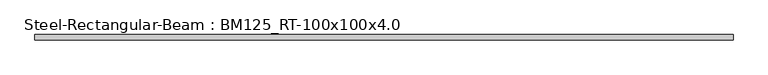
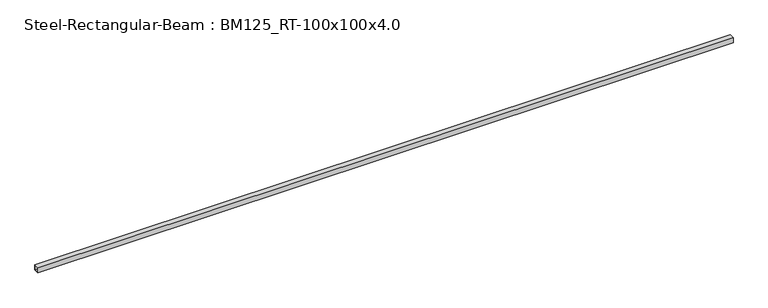
"""IFC4 building model written with IfcOpenShell, lengths in millimetres: beam geometry, Steel-Rectangular-Beam : BM125_RT-100x100x4.0."""

from ifc_helpers import new_model, si_unit, frame, origin, place, context, project, spatial, polyline, outline, extrude, source, transform, mapped, element, save


def steel_rectangular_beam_bm125_rt_100x100x4_0_2c93a6f0(model_context):
    return source(origin(), model_context, "Body", "SweptSolid", [
        extrude(outline(polyline([(-50.0, 50.0), (50.0, 50.0), (50.0, -50.0), (-50.0, -50.0), (-50.0, 50.0)]), holes=[polyline([(46.0, -46.0), (46.0, 46.0), (-46.0, 46.0), (-46.0, -46.0), (46.0, -46.0)])]), frame((-6550.0, 0.0, 0.0), z_axis=(1.0, 0.0, 0.0), x_axis=(0.0, 1.0, 0.0)), (0.0, 0.0, 1.0), 13100.0),
        extrude(outline(polyline([(-50.0, 50.0), (50.0, 50.0), (50.0, -50.0), (-50.0, -50.0), (-50.0, 50.0)]), holes=[polyline([(46.0, -46.0), (46.0, 46.0), (-46.0, 46.0), (-46.0, -46.0), (46.0, -46.0)])]), frame((-6550.0, 0.0, 0.0), z_axis=(1.0, 0.0, 0.0), x_axis=(0.0, 1.0, 0.0)), (0.0, 0.0, 1.0), 13100.0),
        extrude(outline(polyline([(-50.0, 50.0), (50.0, 50.0), (50.0, -50.0), (-50.0, -50.0), (-50.0, 50.0)]), holes=[polyline([(46.0, -46.0), (46.0, 46.0), (-46.0, 46.0), (-46.0, -46.0), (46.0, -46.0)])]), frame((-6550.0, 0.0, 0.0), z_axis=(1.0, 0.0, 0.0), x_axis=(0.0, 1.0, 0.0)), (0.0, 0.0, 1.0), 13100.0),
        extrude(outline(polyline([(-50.0, 50.0), (50.0, 50.0), (50.0, -50.0), (-50.0, -50.0), (-50.0, 50.0)]), holes=[polyline([(46.0, -46.0), (46.0, 46.0), (-46.0, 46.0), (-46.0, -46.0), (46.0, -46.0)])]), frame((-6550.0, 0.0, 0.0), z_axis=(1.0, 0.0, 0.0), x_axis=(0.0, 1.0, 0.0)), (0.0, 0.0, 1.0), 13100.0),
    ])


if __name__ == "__main__":
    model = new_model("IFC4")
    model_context = context("Model", 3, world=origin())
    ifc_project = project(units=[si_unit("LENGTHUNIT", "METRE", prefix="MILLI")], contexts=[model_context])
    site = spatial("IfcSite", under=ifc_project)
    building = spatial("IfcBuilding", under=site)
    placement = place(None, origin())
    steel_rectangular_beam_bm125_rt_100x100x4_0_shape = steel_rectangular_beam_bm125_rt_100x100x4_0_2c93a6f0(model_context)
    element("IfcBeam", 1, ObjectType="Steel-Rectangular-Beam : BM125_RT-100x100x4.0", at=placement, inside=building, context=model_context, shape_type="MappedRepresentation", body=[
        mapped(steel_rectangular_beam_bm125_rt_100x100x4_0_shape, transform((0.0, 0.0, 0.0), x_axis=(1.0, 0.0, 0.0), y_axis=(0.0, 1.0, 0.0), z_axis=(0.0, 0.0, 1.0))),
    ])
    save(model, "model.ifc")

# Revit data of these elements
# Type "Steel-Rectangular-Beam : BM125_RT-100x100x4.0"
#   t = 4 mm
#   Mass per Unit Length = 11.70 kg/m
#   Surface Area = 0.386 m²/m
#   Sectional Area = 14.95 cm²
#   Length [instance default] = 3000 mm
#   H = 100 mm
#   B = 100 mm
#   hec_material4 [instance default] = none
#   hec_material3 [instance default] = none
#   hec_material2 [instance default] = none
#   hec_material1 [instance default] = none
#   Structural Material [instance default] = none
# Element 1 (IfcBeam, "Steel-Rectangular-Beam : BM125_RT-100x100x4.0")
#   hec_material2 = S01AA010-00001_Main Steel Structure Fabrication Work_Shelter/Building_Steel Painting/Coating_for Non-Fireproofed Steel Surface, Surface Preparation, Primer, Second & Final Coat
#   hec_material1 = S03AA007-00001_Main Steel Structure Erection Work_Girth & Purlin
#   Structural Material = S01AA007-00001_Main Steel Structure Fabrication Work_Shelter/Building_Girth & Purlin
#   Materials on its faces: "S01AA010-00001_Main Steel Structure Fabrication Work_Shelter/Building_Steel Painting/Coating_for Non-Fireproofed Steel Surface, Surface Preparation, Primer, Second & Final Coat"
# Materials
#   "S01AA010-00001_Main Steel Structure Fabrication Work_Shelter/Building_Steel Painting/Coating_for Non-Fireproofed Steel Surface, Surface Preparation, Primer, Second & Final Coat": class "Metal", colour RGB 120 120 120, transparency 0, Description = "Paint finished steel", W00) Work Master Code = "S01AA010-00001", W01) Work Master_Lv1 = "Main Steel Structure Fabrication Work", W02) Work Master_Lv2 = "Shelter/Building", W03) Work Master_Spec.1 = "Steel Painting/Coating", W04) Work Master_Spec.2 = "for Non-Fireproofed Steel Surface, Surface Preparation, Primer, Second & Final Coat", Cost = 0
#   "S03AA007-00001_Main Steel Structure Erection Work_Girth & Purlin": class "Metal", colour RGB 120 120 120, transparency 0, Comments = "(30KG/M>Weight)", Description = "Structural steel 50ksi", W00) Work Master Code = "S03AA007-00001", W01) Work Master_Lv1 = "Main Steel Structure Erection Work", W02) Work Master_Lv2 = "Shelter/Building", W03) Work Master_Spec.1 = "Girth & Purlin", Cost = 0
#   "S01AA007-00001_Main Steel Structure Fabrication Work_Shelter/Building_Girth & Purlin": class "Metal", colour RGB 120 120 120, transparency 0, Comments = "(30KG/M>Weight)", Description = "Structural steel 50ksi", W00) Work Master Code = "S01AA007-00001", W01) Work Master_Lv1 = "Main Steel Structure Fabrication Work", W02) Work Master_Lv2 = "Shelter/Building", W03) Work Master_Spec.1 = "Girth & Purlin", Cost = 0
